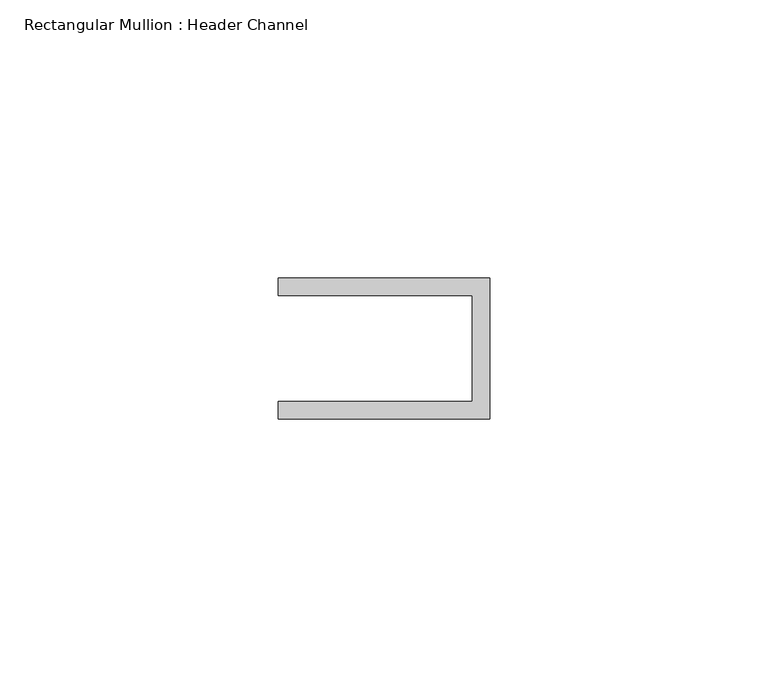
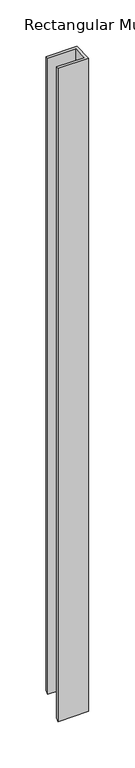
"""IFC4 building model written with IfcOpenShell, lengths in millimetres: member geometry, Rectangular Mullion : Header Channel."""

from ifc_helpers import new_model, si_unit, origin, place, context, project, spatial, faceted_brep, source, transform, mapped, element, save


def rectangular_mullion_header_channel_5370cb82(model_context):
    return source(origin(), model_context, "Body", "Brep", [
        faceted_brep([(0.0, -12.7, 0.0), (0.0, 12.7, 0.0), (-38.1, 12.7, 0.0), (-38.1, 9.525, 0.0), (-3.175, 9.525, 0.0), (-3.175, -9.525, 0.0), (-38.1, -9.525, 0.0), (-38.1, -12.7, 0.0), (0.0, -12.7, -858.1185498), (0.0, 12.7, -832.7185498), (-38.1, 12.7, -832.7185498), (-38.1, 9.525, -835.8935498), (-3.175, 9.525, -835.8935498), (-3.175, -9.525, -854.9435498), (-38.1, -9.525, -854.9435498), (-38.1, -12.7, -858.1185498)], [[[0, 1, 2, 3, 4, 5, 6, 7]], [[1, 0, 8, 9]], [[2, 1, 9, 10]], [[3, 2, 10, 11]], [[4, 3, 11, 12]], [[5, 4, 12, 13]], [[6, 5, 13, 14]], [[7, 6, 14, 15]], [[0, 7, 15, 8]], [[8, 15, 14, 13, 12, 11, 10, 9]]]),
    ])


if __name__ == "__main__":
    model = new_model("IFC4")
    model_context = context("Model", 3, world=origin())
    ifc_project = project(units=[si_unit("LENGTHUNIT", "METRE", prefix="MILLI")], contexts=[model_context])
    site = spatial("IfcSite", under=ifc_project)
    building = spatial("IfcBuilding", under=site)
    placement = place(None, origin())
    rectangular_mullion_header_channel_shape = rectangular_mullion_header_channel_5370cb82(model_context)
    element("IfcMember", 1, ObjectType="Rectangular Mullion : Header Channel", at=placement, inside=building, context=model_context, shape_type="MappedRepresentation", body=[
        mapped(rectangular_mullion_header_channel_shape, transform((0.0, 0.0, 0.0), x_axis=(1.0, 0.0, 0.0), y_axis=(0.0, 1.0, 0.0), z_axis=(0.0, 0.0, 1.0))),
    ])
    save(model, "model.ifc")

# Revit data of these elements
# Type "Rectangular Mullion : Header Channel"
#   built-in parameter 1007322 = 0.0833333 (stored number, unit not read)
#   built-in parameter 1007321 = -0.03125 (stored number, unit not read)
#   built-in parameter 1007320 = 0.0416667 (stored number, unit not read)
# Element 1 (IfcMember, "Rectangular Mullion : Header Channel")
#   Materials on its faces: "ALUM"
# Materials
#   "ALUM": class "Generic", colour RGB 157 157 157, transparency 0, Cost = 0
